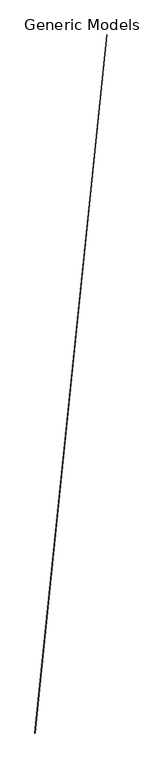
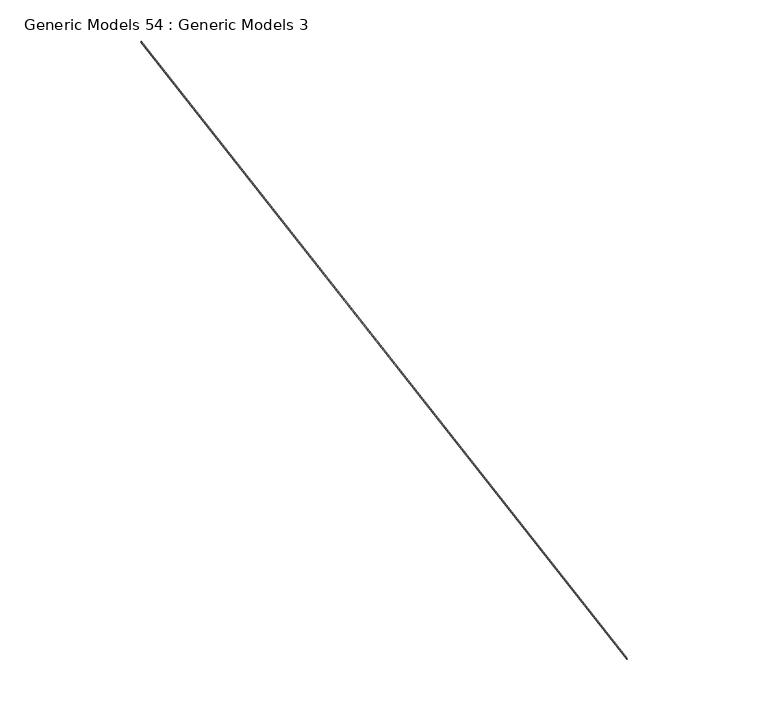
"""IFC4 building model written with IfcOpenShell, lengths in millimetres: proxy geometry, Generic Models 54 : Generic Models 3."""

import ifcopenshell
import ifcopenshell.guid

model = None  # the IFC model being written
_history = None  # IfcOwnerHistory: only IFC2X3 demands one
_inside = {}  # id of a spatial element -> (the spatial element, [elements in it])
_under = {}  # id of a project, library or spatial element -> (it, [spatial elements below it])
_declared = {}  # id of a project -> (the project, [libraries it declares])
_typed = {}  # id of a type object -> (the type object, [elements of that type])
_made_of = {}  # id of a material, layer set ... -> (it, [elements and type objects made of it])


def new_model(schema):
    """Start an empty IFC model of exactly this schema.

    Asked for "IFC4X3", IfcOpenShell would pick the latest addendum, in which some entities
    have other attributes; the version numbers below select the first issue.
    IFC2X3 requires an IfcOwnerHistory on every rooted entity: one is made here for all.
    """
    global model, _history
    if schema == "IFC4X3":
        model = ifcopenshell.file(schema_version=(4, 3, 0, 0))
    else:
        model = ifcopenshell.file(schema=schema)
    _inside.clear()
    _under.clear()
    _declared.clear()
    _typed.clear()
    _made_of.clear()
    _history = None
    if model.schema == "IFC2X3":
        org = make("IfcOrganization", Name="unknown")
        user = make(
            "IfcPersonAndOrganization",
            ThePerson=make("IfcPerson", FamilyName="unknown"),
            TheOrganization=org,
        )
        app = make(
            "IfcApplication",
            ApplicationDeveloper=org,
            Version="unknown",
            ApplicationFullName="unknown",
            ApplicationIdentifier="unknown",
        )
        _history = make(
            "IfcOwnerHistory",
            OwningUser=user,
            OwningApplication=app,
            ChangeAction="ADDED",
            CreationDate=0,
        )
    return model


def make(cls, **values):
    """One entity of the class cls with the attributes given. An attribute that is None is left unset."""
    return model.create_entity(
        cls, **{name: value for name, value in values.items() if value is not None}
    )


def rooted(cls, **values):
    """An entity with a GlobalId (a new one), such as an element, a storey or a relation."""
    return make(cls, GlobalId=ifcopenshell.guid.new(), OwnerHistory=_history, **values)


def si_unit(unit_type, name, prefix=None):
    """IfcSIUnit, for example si_unit("LENGTHUNIT", "METRE", prefix="MILLI")."""
    return make("IfcSIUnit", UnitType=unit_type, Prefix=prefix, Name=name)


def assignment(units):
    """IfcUnitAssignment: the units of a project."""
    return None if units is None else make("IfcUnitAssignment", Units=units)


def point(xyz):
    """IfcCartesianPoint."""
    return None if xyz is None else make("IfcCartesianPoint", Coordinates=xyz)


def direction(xyz):
    """IfcDirection."""
    return None if xyz is None else make("IfcDirection", DirectionRatios=xyz)


def frame(location, z_axis=None, x_axis=None):
    """IfcAxis2Placement3D, a coordinate frame: its origin and axes. An axis left out is left unset."""
    return make(
        "IfcAxis2Placement3D",
        Location=point(location),
        Axis=direction(z_axis),
        RefDirection=direction(x_axis),
    )


def origin():
    """The frame at (0, 0, 0) with its axes left unset."""
    return frame((0.0, 0.0, 0.0))


def place(relative_to, where):
    """IfcLocalPlacement: puts the frame where relative to a parent placement (None: the world)."""
    return make(
        "IfcLocalPlacement", PlacementRelTo=relative_to, RelativePlacement=where
    )


def context(
    kind, dimensions, precision=None, world=None, true_north=None, identifier=None
):
    """IfcGeometricRepresentationContext, for example the 3D "Model" context."""
    return make(
        "IfcGeometricRepresentationContext",
        ContextIdentifier=identifier,
        ContextType=kind,
        CoordinateSpaceDimension=dimensions,
        Precision=precision,
        WorldCoordinateSystem=world,
        TrueNorth=true_north,
    )


def project(units=None, contexts=None):
    """IfcProject with its units and contexts."""
    return rooted(
        "IfcProject",
        Name="project",
        RepresentationContexts=contexts,
        UnitsInContext=assignment(units),
    )


def spatial(cls, under=None, at=None, **own):
    """A site, building, storey or space (cls), placed at a placement, below another one or the project."""
    s = rooted(cls, ObjectPlacement=at, **own)
    if under is not None:
        _under.setdefault(under.id(), (under, []))[1].append(s)
    return s


def polyline(points):
    """IfcPolyline through the points."""
    return make("IfcPolyline", Points=[point(p) for p in points])


def outline(outer, holes=None, kind="AREA"):
    """IfcArbitraryClosedProfileDef: a profile drawn as a closed curve; with holes, ...WithVoids."""
    if holes is None:
        return make("IfcArbitraryClosedProfileDef", ProfileType=kind, OuterCurve=outer)
    return make(
        "IfcArbitraryProfileDefWithVoids",
        ProfileType=kind,
        OuterCurve=outer,
        InnerCurves=holes,
    )


def extrude(swept, where, along, depth):
    """IfcExtrudedAreaSolid: the profile swept, set in the frame where, extruded along a direction by depth."""
    return make(
        "IfcExtrudedAreaSolid",
        SweptArea=swept,
        Position=where,
        ExtrudedDirection=direction(along),
        Depth=depth,
    )


def shape(context_of_items, identifier, shape_type, items):
    """IfcShapeRepresentation: the items that make up one representation, for example the "Body"."""
    return make(
        "IfcShapeRepresentation",
        ContextOfItems=context_of_items,
        RepresentationIdentifier=identifier,
        RepresentationType=shape_type,
        Items=items,
    )


def source(mapping_origin, context_of_items, identifier, shape_type, items):
    """IfcRepresentationMap: a shape defined once, which mapped items show again and again."""
    return make(
        "IfcRepresentationMap",
        MappingOrigin=mapping_origin,
        MappedRepresentation=shape(context_of_items, identifier, shape_type, items),
    )


def transform(
    local_origin,
    x_axis=None,
    y_axis=None,
    z_axis=None,
    scale=None,
    scale2=None,
    scale3=None,
    uniform=True,
):
    """IfcCartesianTransformationOperator3D, or its non-uniform kind. x_axis, y_axis, z_axis: its Axis1, 2, 3."""
    if uniform:
        return make(
            "IfcCartesianTransformationOperator3D",
            Axis1=direction(x_axis),
            Axis2=direction(y_axis),
            LocalOrigin=point(local_origin),
            Scale=scale,
            Axis3=direction(z_axis),
        )
    return make(
        "IfcCartesianTransformationOperator3DnonUniform",
        Axis1=direction(x_axis),
        Axis2=direction(y_axis),
        LocalOrigin=point(local_origin),
        Scale=scale,
        Axis3=direction(z_axis),
        Scale2=scale2,
        Scale3=scale3,
    )


def mapped(mapping_source, mapping_target):
    """IfcMappedItem: shows the shape of a source again, moved by a transform."""
    return make(
        "IfcMappedItem", MappingSource=mapping_source, MappingTarget=mapping_target
    )


def made_of(thing, what):
    """Note that an element or type object is made of a material, layer set ...; save() writes the relation."""
    if what is not None:
        _made_of.setdefault(what.id(), (what, []))[1].append(thing)
    return thing


def element(
    cls,
    number,
    at=None,
    inside=None,
    cuts=None,
    type_object=None,
    material=None,
    context=None,
    identifier="Body",
    shape_type=None,
    held_by="IfcProductDefinitionShape",
    body=None,
    shapes=None,
    **own,
):
    """One element of the class cls, such as IfcWall. Its Tag is "e" and its number.

    at: its placement. inside: the storey or other place that contains it. cuts: it is an
    opening in that element (IfcRelVoidsElement). A single representation is given by context,
    identifier, shape_type and body (its items); several are given by shapes. held_by: the class
    of the entity that holds the representations. save() writes the other relations.
    """
    e = rooted(cls, Tag="e%d" % number, ObjectPlacement=at, **own)
    if body is not None:
        shapes = [shape(context, identifier, shape_type, body)]
    if shapes is not None:
        e.Representation = make(held_by, Representations=shapes)
    if inside is not None:
        _inside.setdefault(inside.id(), (inside, []))[1].append(e)
    if cuts is not None:
        rooted(
            "IfcRelVoidsElement", RelatingBuildingElement=cuts, RelatedOpeningElement=e
        )
    if type_object is not None:
        _typed.setdefault(type_object.id(), (type_object, []))[1].append(e)
    return made_of(e, material)


def aggregate(whole, parts):
    """IfcRelAggregates: a whole, such as a stair, and the parts it consists of."""
    return rooted("IfcRelAggregates", RelatingObject=whole, RelatedObjects=parts)


def save(model, path):
    """Write the relations noted so far, then the file.

    IfcRelAggregates (storeys below a building ...), IfcRelContainedInSpatialStructure (elements
    in a storey), IfcRelDefinesByType, IfcRelAssociatesMaterial and IfcRelDeclares: one each for
    every whole, place, type object, material and project.
    """
    for whole, parts in _under.values():
        aggregate(whole, parts)
    for where, things in _inside.values():
        rooted(
            "IfcRelContainedInSpatialStructure",
            RelatedElements=things,
            RelatingStructure=where,
        )
    for kind, things in _typed.values():
        rooted("IfcRelDefinesByType", RelatedObjects=things, RelatingType=kind)
    for what, things in _made_of.values():
        rooted("IfcRelAssociatesMaterial", RelatedObjects=things, RelatingMaterial=what)
    for by, libraries in _declared.values():
        rooted("IfcRelDeclares", RelatingContext=by, RelatedDefinitions=libraries)
    model.write(path)


def generic_models_54_generic_models_3_cbdb2cac(model_context):
    return source(origin(), model_context, "Body", "SweptSolid", [
        extrude(outline(polyline([(87.7086854, 0.0), (87.7086854, -17.0540674), (93.5851851, -22.2356445), (92.5352676, -23.4263709), (86.1211853, -17.770783), (86.1211854, 0.0), (87.7086854, 0.0)])), frame((35322.91049, 40694.2893712, 272175.800179), z_axis=(-0.10293344407674773, -0.9946674410191907, 0.006433340254794665), x_axis=(0.9926875075994102, -0.10313426588887777, -0.06272826679921324)), (0.0, 0.0, 1.0), 15089.019704),
    ])


if __name__ == "__main__":
    model = new_model("IFC4")
    model_context = context("Model", 3, world=origin())
    ifc_project = project(units=[si_unit("LENGTHUNIT", "METRE", prefix="MILLI")], contexts=[model_context])
    site = spatial("IfcSite", under=ifc_project)
    building = spatial("IfcBuilding", under=site)
    placement = place(None, origin())
    generic_models_54_generic_models_3_shape = generic_models_54_generic_models_3_cbdb2cac(model_context)
    element("IfcBuildingElementProxy", 1, Name="Generic Models 54 : Generic Models 3", ObjectType="Generic Models 54 : Generic Models 3", at=placement, inside=building, context=model_context, shape_type="MappedRepresentation", body=[
        mapped(generic_models_54_generic_models_3_shape, transform((0.0, 0.0, 0.0), x_axis=(1.0, 0.0, 0.0), y_axis=(0.0, 1.0, 0.0), z_axis=(0.0, 0.0, 1.0))),
    ])
    save(model, "model.ifc")

# Revit data of these elements
# Element 1 (IfcBuildingElementProxy, "Generic Models 54 : Generic Models 3")
#   Materials on its faces: "SEAMLESS CONCEALED SHEET METAL GUTTER - (COLOR: EXTRA DARK BRONZE)"
# Materials
#   "SEAMLESS CONCEALED SHEET METAL GUTTER - (COLOR: EXTRA DARK BRONZE)": class "Generic", colour RGB 97 74 67, transparency 0, Cost = 0
